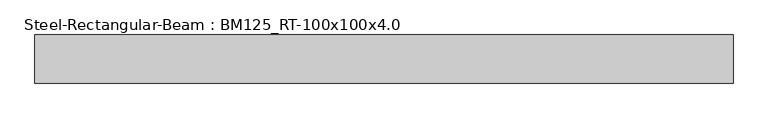
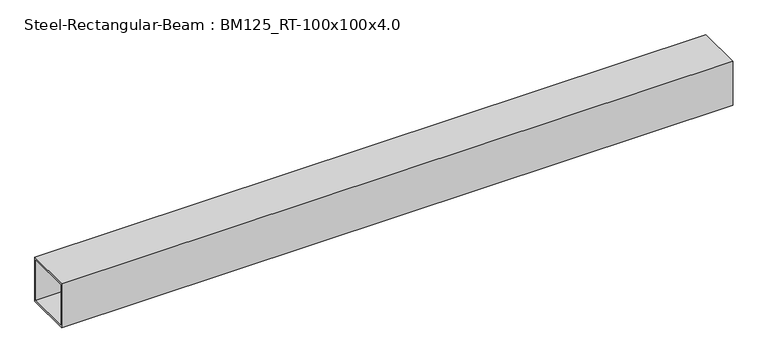
"""IFC4 building model written with IfcOpenShell, lengths in millimetres: beam geometry, Steel-Rectangular-Beam : BM125_RT-100x100x4.0."""

from ifc_helpers import new_model, si_unit, frame, origin, place, context, project, spatial, polyline, outline, extrude, source, transform, mapped, element, save


def steel_rectangular_beam_bm125_rt_100x100x4_0_366960fc(model_context):
    return source(origin(), model_context, "Body", "SweptSolid", [
        extrude(outline(polyline([(-50.0, 50.0), (50.0, 50.0), (50.0, -50.0), (-50.0, -50.0), (-50.0, 50.0)]), holes=[polyline([(46.0, -46.0), (46.0, 46.0), (-46.0, 46.0), (-46.0, -46.0), (46.0, -46.0)])]), frame((-725.0, 0.0, 0.0), z_axis=(1.0, 0.0, 0.0), x_axis=(0.0, 1.0, 0.0)), (0.0, 0.0, 1.0), 1450.0),
        extrude(outline(polyline([(-50.0, 50.0), (50.0, 50.0), (50.0, -50.0), (-50.0, -50.0), (-50.0, 50.0)]), holes=[polyline([(46.0, -46.0), (46.0, 46.0), (-46.0, 46.0), (-46.0, -46.0), (46.0, -46.0)])]), frame((-725.0, 0.0, 0.0), z_axis=(1.0, 0.0, 0.0), x_axis=(0.0, 1.0, 0.0)), (0.0, 0.0, 1.0), 1450.0),
        extrude(outline(polyline([(-50.0, 50.0), (50.0, 50.0), (50.0, -50.0), (-50.0, -50.0), (-50.0, 50.0)]), holes=[polyline([(46.0, -46.0), (46.0, 46.0), (-46.0, 46.0), (-46.0, -46.0), (46.0, -46.0)])]), frame((-725.0, 0.0, 0.0), z_axis=(1.0, 0.0, 0.0), x_axis=(0.0, 1.0, 0.0)), (0.0, 0.0, 1.0), 1450.0),
        extrude(outline(polyline([(-50.0, 50.0), (50.0, 50.0), (50.0, -50.0), (-50.0, -50.0), (-50.0, 50.0)]), holes=[polyline([(46.0, -46.0), (46.0, 46.0), (-46.0, 46.0), (-46.0, -46.0), (46.0, -46.0)])]), frame((-725.0, 0.0, 0.0), z_axis=(1.0, 0.0, 0.0), x_axis=(0.0, 1.0, 0.0)), (0.0, 0.0, 1.0), 1450.0),
    ])


if __name__ == "__main__":
    model = new_model("IFC4")
    model_context = context("Model", 3, world=origin())
    ifc_project = project(units=[si_unit("LENGTHUNIT", "METRE", prefix="MILLI")], contexts=[model_context])
    site = spatial("IfcSite", under=ifc_project)
    building = spatial("IfcBuilding", under=site)
    placement = place(None, origin())
    steel_rectangular_beam_bm125_rt_100x100x4_0_shape = steel_rectangular_beam_bm125_rt_100x100x4_0_366960fc(model_context)
    element("IfcBeam", 1, ObjectType="Steel-Rectangular-Beam : BM125_RT-100x100x4.0", at=placement, inside=building, context=model_context, shape_type="MappedRepresentation", body=[
        mapped(steel_rectangular_beam_bm125_rt_100x100x4_0_shape, transform((0.0, 0.0, 0.0), x_axis=(1.0, 0.0, 0.0), y_axis=(0.0, 1.0, 0.0), z_axis=(0.0, 0.0, 1.0))),
    ])
    save(model, "model.ifc")

# Revit data of these elements
# Type "Steel-Rectangular-Beam : BM125_RT-100x100x4.0"
#   t = 4 mm
#   Mass per Unit Length = 11.70 kg/m
#   Surface Area = 0.386 m²/m
#   Sectional Area = 14.95 cm²
#   Length [instance default] = 3000 mm
#   H = 100 mm
#   B = 100 mm
#   hec_material4 [instance default] = none
#   hec_material3 [instance default] = none
#   hec_material2 [instance default] = none
#   hec_material1 [instance default] = none
#   Structural Material [instance default] = none
# Element 1 (IfcBeam, "Steel-Rectangular-Beam : BM125_RT-100x100x4.0")
#   hec_material2 = S01AA010-00001_Main Steel Structure Fabrication Work_Shelter/Building_Steel Painting/Coating_for Non-Fireproofed Steel Surface, Surface Preparation, Primer, Second & Final Coat
#   hec_material1 = S03AA007-00001_Main Steel Structure Erection Work_Girth & Purlin
#   Structural Material = S01AA007-00001_Main Steel Structure Fabrication Work_Shelter/Building_Girth & Purlin
#   Materials on its faces: "S01AA010-00001_Main Steel Structure Fabrication Work_Shelter/Building_Steel Painting/Coating_for Non-Fireproofed Steel Surface, Surface Preparation, Primer, Second & Final Coat"
# Materials
#   "S01AA010-00001_Main Steel Structure Fabrication Work_Shelter/Building_Steel Painting/Coating_for Non-Fireproofed Steel Surface, Surface Preparation, Primer, Second & Final Coat": class "Metal", colour RGB 120 120 120, transparency 0, Description = "Paint finished steel", W00) Work Master Code = "S01AA010-00001", W01) Work Master_Lv1 = "Main Steel Structure Fabrication Work", W02) Work Master_Lv2 = "Shelter/Building", W03) Work Master_Spec.1 = "Steel Painting/Coating", W04) Work Master_Spec.2 = "for Non-Fireproofed Steel Surface, Surface Preparation, Primer, Second & Final Coat", Cost = 0
#   "S03AA007-00001_Main Steel Structure Erection Work_Girth & Purlin": class "Metal", colour RGB 120 120 120, transparency 0, Comments = "(30KG/M>Weight)", Description = "Structural steel 50ksi", W00) Work Master Code = "S03AA007-00001", W01) Work Master_Lv1 = "Main Steel Structure Erection Work", W02) Work Master_Lv2 = "Shelter/Building", W03) Work Master_Spec.1 = "Girth & Purlin", Cost = 0
#   "S01AA007-00001_Main Steel Structure Fabrication Work_Shelter/Building_Girth & Purlin": class "Metal", colour RGB 120 120 120, transparency 0, Comments = "(30KG/M>Weight)", Description = "Structural steel 50ksi", W00) Work Master Code = "S01AA007-00001", W01) Work Master_Lv1 = "Main Steel Structure Fabrication Work", W02) Work Master_Lv2 = "Shelter/Building", W03) Work Master_Spec.1 = "Girth & Purlin", Cost = 0
